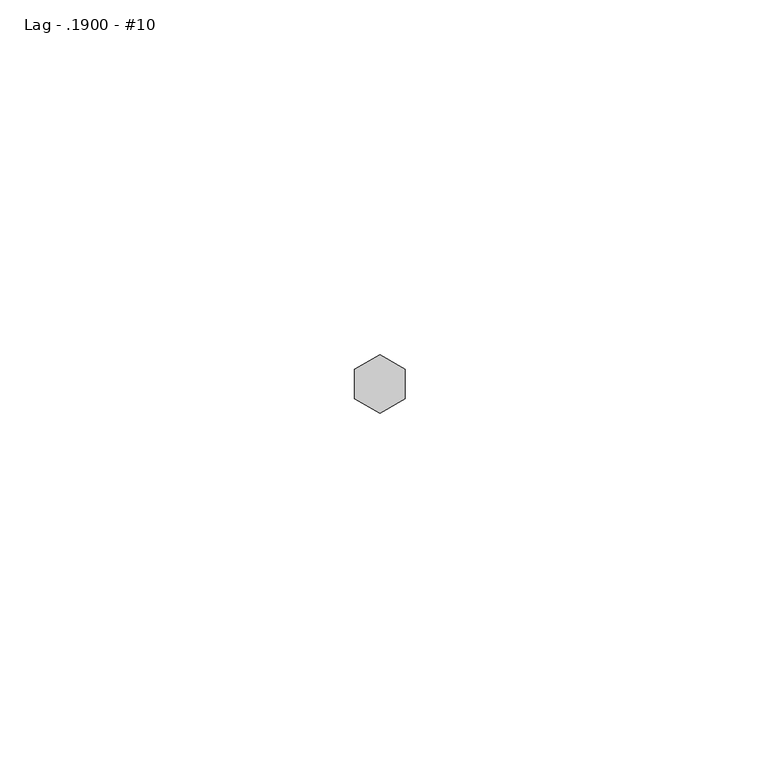
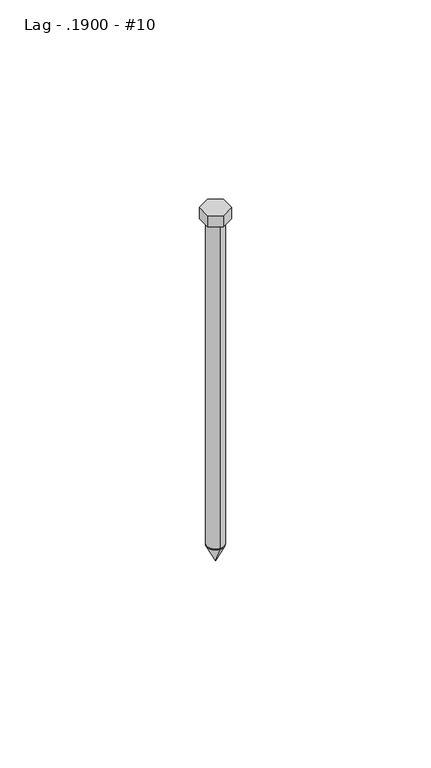
"""IFC4 building model written with IfcOpenShell, lengths in millimetres: fastener geometry, 060523 - W_P_C - Fastenings - Generic : Lag - .1900 - #10."""

from ifc_helpers import new_model, si_unit, point, frame, origin, origin_with_axes, origin_2d, place, context, project, spatial, polyline, circle_curve, trimmed, segment, composite_curve, outline, extrude, source, transform, mapped, element, save
from ifc_brep_helpers import plane_surface, revolved_surface, advanced_brep


def lag_1900_10_4b50847c(model_context):
    return source(origin(), model_context, "Body", "SolidModel", [
        advanced_brep(
        [(0.0, -2.5300781, -101.6), (0.0, 2.5300781, -101.6), (0.0, 0.0, -101.6), (0.0, 0.0, -106.6601562)],
        [
            (0, 1, circle_curve(frame((0.0, 0.0, -101.6), z_axis=(0.0, 0.0, 1.0), x_axis=(0.0, 1.0, 0.0)), 2.5300781)),
            (1, 2),
            (2, 0),
            (1, 0, circle_curve(frame((0.0, 0.0, -101.6), z_axis=(0.0, 0.0, 1.0), x_axis=(0.0, 1.0, 0.0)), 2.5300781)),
            (3, 1),
            (0, 3),
        ],
        [
            plane_surface(frame((0.0, 0.0, -101.6), z_axis=(0.0, 0.0, 1.0), x_axis=(0.0, 1.0, 0.0))),
            revolved_surface(polyline([(0.0, 2.5300781, -101.6), (0.0, 0.0, -106.6601562)]), (0.0, 0.0, -103.0840259), (0.0, 0.0, -1.0)),
        ],
        [
            (0, [[1, 2, 3]]),
            (0, [[4, -3, -2]]),
            (1, [[5, -1, 6]]),
            (1, [[-6, -4, -5]]),
        ],
    ),
        extrude(outline(polyline([(-3.571875, 2.062223), (0.0, 4.124446), (3.571875, 2.062223), (3.571875, -2.062223), (0.0, -4.124446), (-3.571875, -2.062223), (-3.571875, 2.062223)])), origin_with_axes(), (0.0, 0.0, 1.0), 3.571875),
        extrude(outline(composite_curve([segment(trimmed(circle_curve(origin_2d(), 2.5300781), [point((0.0, -2.5300781))], [point((0.0, 2.5300781))], False, "CARTESIAN"), True, "CONTINUOUS"), segment(trimmed(circle_curve(origin_2d(), 2.5300781), [point((0.0, 2.5300781))], [point((0.0, -2.5300781))], False, "CARTESIAN"), True, "CONTINUOUS")], self_intersect=False)), frame((0.0, 0.0, -101.6), z_axis=(0.0, 0.0, 1.0), x_axis=(1.0, 0.0, 0.0)), (0.0, 0.0, 1.0), 101.6),
    ])


if __name__ == "__main__":
    model = new_model("IFC4")
    model_context = context("Model", 3, world=origin())
    ifc_project = project(units=[si_unit("LENGTHUNIT", "METRE", prefix="MILLI")], contexts=[model_context])
    site = spatial("IfcSite", under=ifc_project)
    building = spatial("IfcBuilding", under=site)
    placement = place(None, origin())
    lag_1900_10_shape = lag_1900_10_4b50847c(model_context)
    element("IfcFastener", 1, ObjectType="060523 - W_P_C - Fastenings - Generic : Lag - .1900 - #10", at=placement, inside=building, context=model_context, shape_type="MappedRepresentation", body=[
        mapped(lag_1900_10_shape, transform((0.0, 0.0, 0.0), x_axis=(1.0, 0.0, 0.0), y_axis=(0.0, 1.0, 0.0), z_axis=(0.0, 0.0, 1.0))),
    ])
    save(model, "model.ifc")

# Revit data of these elements
# Type "060523 - W_P_C - Fastenings - Generic : Lag - .1900 - #10"
#   Washer_Thickness = 0' - 0 3/64"
#   Washer Radius = 0' - 0.24023"
#   Washer Offset - Head = 0' - 0"
#   Washer Offset = 0' - 0"
#   Thickness_of_Substrate [instance default] = 0' - 1"
#   Side = 0' - 0.1626"
#   Radius = 0' - 0.09961"
#   Length [instance default] = 0' - 4"
#   Head Size = 0' - 0 9/32"
#   Head Radius = 0' - 0 9/64"
#   Head Height = 0' - 0 9/64"
#   Double Diameter = 0' - 0 51/128"
#   Diameter = 0' - 0 51/256"
#   Default Elevation = 4' - 0"
#   Washer_Nut_Visibility = no
#   Washer_Head_Visibility = no
#   Round_Head_Visibility = no
#   Point Visibility = yes
#   Nut_Visibility = no
#   Hex_Head_Visiblilty = yes
#   Washer Material = none
#   Bolt Material (Size) = AT SILL - FASTENER AT 24" O.C.
# Element 1 (IfcFastener, "060523 - W_P_C - Fastenings - Generic : Lag - .1900 - #10")
#   Materials on its faces: "AT SILL - FASTENER AT 24\" O.C."
# Materials
#   "AT SILL - FASTENER AT 24\" O.C.": class "Generic", colour RGB 120 120 120, transparency 0, Cost = 0
